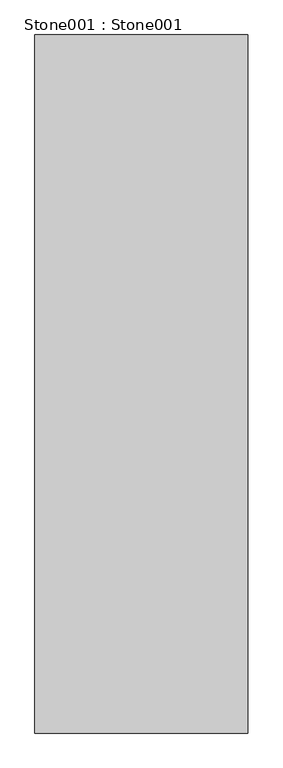
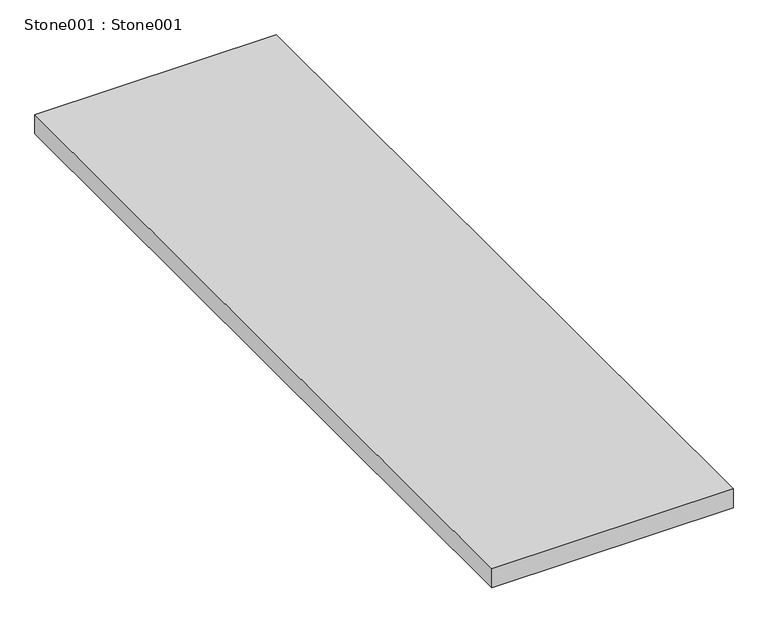
"""IFC4 building model written with IfcOpenShell, lengths in millimetres: proxy geometry, Stone001 : Stone001."""

from ifc_helpers import new_model, si_unit, frame, origin, place, context, project, spatial, polyline, outline, extrude, source, transform, mapped, element, save


def stone001_stone001_bd3c5613(model_context):
    return source(origin(), model_context, "Body", "SweptSolid", [
        extrude(outline(polyline([(-4877.6505001, -1052.8906574), (-5487.2505001, -1052.8906574), (-5487.2505001, 947.1093426), (-4877.6505001, 947.1093426), (-4877.6505001, -1052.8906574)])), frame((0.0, 0.0, 36508.2444375), z_axis=(0.0, 0.0, 1.0), x_axis=(1.0, 0.0, 0.0)), (0.0, 0.0, 1.0), 50.8),
    ])


if __name__ == "__main__":
    model = new_model("IFC4")
    model_context = context("Model", 3, world=origin())
    ifc_project = project(units=[si_unit("LENGTHUNIT", "METRE", prefix="MILLI")], contexts=[model_context])
    site = spatial("IfcSite", under=ifc_project)
    building = spatial("IfcBuilding", under=site)
    placement = place(None, origin())
    stone001_stone001_shape = stone001_stone001_bd3c5613(model_context)
    element("IfcBuildingElementProxy", 1, Name="Stone001 : Stone001", ObjectType="Stone001 : Stone001", at=placement, inside=building, context=model_context, shape_type="MappedRepresentation", body=[
        mapped(stone001_stone001_shape, transform((0.0, 0.0, 0.0), x_axis=(1.0, 0.0, 0.0), y_axis=(0.0, 1.0, 0.0), z_axis=(0.0, 0.0, 1.0))),
    ])
    save(model, "model.ifc")

# Revit data of these elements
# Type "Stone001 : Stone001"
#   NameOverride = "Stone001"
# Element 1 (IfcBuildingElementProxy, "Stone001 : Stone001")
#   Materials on its faces: "2\" STONE DECK TBD"
# Materials
#   "2\" STONE DECK TBD": class "Unassigned", colour RGB 199 185 173, transparency 0
